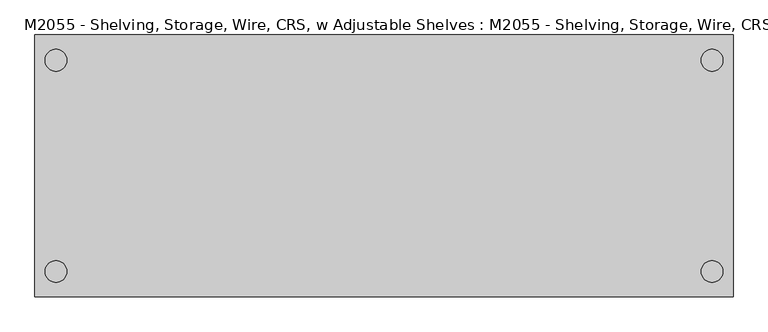
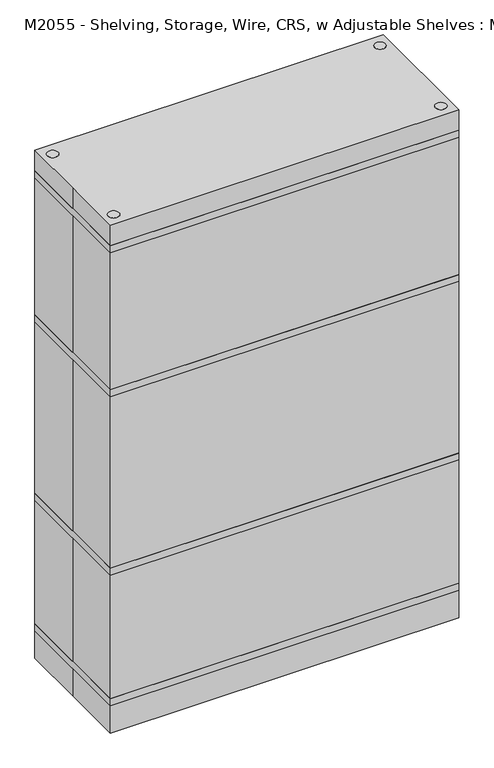
"""IFC4 building model written with IfcOpenShell, lengths in millimetres: proxy geometry, M2055 - Shelving, Storage, Wire, CRS, w Adjustable Shelves : M2055 - Shelving, Storage, Wire, CRS, w Adjustable Shelves."""

import ifcopenshell
import ifcopenshell.guid

model = None  # the IFC model being written
_history = None  # IfcOwnerHistory: only IFC2X3 demands one
_inside = {}  # id of a spatial element -> (the spatial element, [elements in it])
_under = {}  # id of a project, library or spatial element -> (it, [spatial elements below it])
_declared = {}  # id of a project -> (the project, [libraries it declares])
_typed = {}  # id of a type object -> (the type object, [elements of that type])
_made_of = {}  # id of a material, layer set ... -> (it, [elements and type objects made of it])


def new_model(schema):
    """Start an empty IFC model of exactly this schema.

    Asked for "IFC4X3", IfcOpenShell would pick the latest addendum, in which some entities
    have other attributes; the version numbers below select the first issue.
    IFC2X3 requires an IfcOwnerHistory on every rooted entity: one is made here for all.
    """
    global model, _history
    if schema == "IFC4X3":
        model = ifcopenshell.file(schema_version=(4, 3, 0, 0))
    else:
        model = ifcopenshell.file(schema=schema)
    _inside.clear()
    _under.clear()
    _declared.clear()
    _typed.clear()
    _made_of.clear()
    _history = None
    if model.schema == "IFC2X3":
        org = make("IfcOrganization", Name="unknown")
        user = make(
            "IfcPersonAndOrganization",
            ThePerson=make("IfcPerson", FamilyName="unknown"),
            TheOrganization=org,
        )
        app = make(
            "IfcApplication",
            ApplicationDeveloper=org,
            Version="unknown",
            ApplicationFullName="unknown",
            ApplicationIdentifier="unknown",
        )
        _history = make(
            "IfcOwnerHistory",
            OwningUser=user,
            OwningApplication=app,
            ChangeAction="ADDED",
            CreationDate=0,
        )
    return model


def make(cls, **values):
    """One entity of the class cls with the attributes given. An attribute that is None is left unset."""
    return model.create_entity(
        cls, **{name: value for name, value in values.items() if value is not None}
    )


def rooted(cls, **values):
    """An entity with a GlobalId (a new one), such as an element, a storey or a relation."""
    return make(cls, GlobalId=ifcopenshell.guid.new(), OwnerHistory=_history, **values)


def si_unit(unit_type, name, prefix=None):
    """IfcSIUnit, for example si_unit("LENGTHUNIT", "METRE", prefix="MILLI")."""
    return make("IfcSIUnit", UnitType=unit_type, Prefix=prefix, Name=name)


def assignment(units):
    """IfcUnitAssignment: the units of a project."""
    return None if units is None else make("IfcUnitAssignment", Units=units)


def point(xyz):
    """IfcCartesianPoint."""
    return None if xyz is None else make("IfcCartesianPoint", Coordinates=xyz)


def direction(xyz):
    """IfcDirection."""
    return None if xyz is None else make("IfcDirection", DirectionRatios=xyz)


def frame(location, z_axis=None, x_axis=None):
    """IfcAxis2Placement3D, a coordinate frame: its origin and axes. An axis left out is left unset."""
    return make(
        "IfcAxis2Placement3D",
        Location=point(location),
        Axis=direction(z_axis),
        RefDirection=direction(x_axis),
    )


def frame_2d(location, x_axis=None):
    """IfcAxis2Placement2D, a coordinate frame in the plane: its origin and x axis."""
    return make(
        "IfcAxis2Placement2D", Location=point(location), RefDirection=direction(x_axis)
    )


def origin():
    """The frame at (0, 0, 0) with its axes left unset."""
    return frame((0.0, 0.0, 0.0))


def origin_with_axes():
    """The frame at (0, 0, 0) with the z axis (0, 0, 1) and the x axis (1, 0, 0) written out."""
    return frame((0.0, 0.0, 0.0), z_axis=(0.0, 0.0, 1.0), x_axis=(1.0, 0.0, 0.0))


def place(relative_to, where):
    """IfcLocalPlacement: puts the frame where relative to a parent placement (None: the world)."""
    return make(
        "IfcLocalPlacement", PlacementRelTo=relative_to, RelativePlacement=where
    )


def context(
    kind, dimensions, precision=None, world=None, true_north=None, identifier=None
):
    """IfcGeometricRepresentationContext, for example the 3D "Model" context."""
    return make(
        "IfcGeometricRepresentationContext",
        ContextIdentifier=identifier,
        ContextType=kind,
        CoordinateSpaceDimension=dimensions,
        Precision=precision,
        WorldCoordinateSystem=world,
        TrueNorth=true_north,
    )


def project(units=None, contexts=None):
    """IfcProject with its units and contexts."""
    return rooted(
        "IfcProject",
        Name="project",
        RepresentationContexts=contexts,
        UnitsInContext=assignment(units),
    )


def spatial(cls, under=None, at=None, **own):
    """A site, building, storey or space (cls), placed at a placement, below another one or the project."""
    s = rooted(cls, ObjectPlacement=at, **own)
    if under is not None:
        _under.setdefault(under.id(), (under, []))[1].append(s)
    return s


def polyline(points):
    """IfcPolyline through the points."""
    return make("IfcPolyline", Points=[point(p) for p in points])


def circle_curve(where, radius):
    """IfcCircle in the frame where."""
    return make("IfcCircle", Position=where, Radius=radius)


def trimmed(basis, trim1, trim2, sense, master):
    """IfcTrimmedCurve: the piece of a basis curve between two trims."""
    return make(
        "IfcTrimmedCurve",
        BasisCurve=basis,
        Trim1=trim1,
        Trim2=trim2,
        SenseAgreement=sense,
        MasterRepresentation=master,
    )


def segment(curve, same_sense, transition):
    """IfcCompositeCurveSegment."""
    return make(
        "IfcCompositeCurveSegment",
        Transition=transition,
        SameSense=same_sense,
        ParentCurve=curve,
    )


def composite_curve(segments, self_intersect=None):
    """IfcCompositeCurve: segments joined end to end."""
    return make("IfcCompositeCurve", Segments=segments, SelfIntersect=self_intersect)


def outline(outer, holes=None, kind="AREA"):
    """IfcArbitraryClosedProfileDef: a profile drawn as a closed curve; with holes, ...WithVoids."""
    if holes is None:
        return make("IfcArbitraryClosedProfileDef", ProfileType=kind, OuterCurve=outer)
    return make(
        "IfcArbitraryProfileDefWithVoids",
        ProfileType=kind,
        OuterCurve=outer,
        InnerCurves=holes,
    )


def extrude(swept, where, along, depth):
    """IfcExtrudedAreaSolid: the profile swept, set in the frame where, extruded along a direction by depth."""
    return make(
        "IfcExtrudedAreaSolid",
        SweptArea=swept,
        Position=where,
        ExtrudedDirection=direction(along),
        Depth=depth,
    )


def shape(context_of_items, identifier, shape_type, items):
    """IfcShapeRepresentation: the items that make up one representation, for example the "Body"."""
    return make(
        "IfcShapeRepresentation",
        ContextOfItems=context_of_items,
        RepresentationIdentifier=identifier,
        RepresentationType=shape_type,
        Items=items,
    )


def source(mapping_origin, context_of_items, identifier, shape_type, items):
    """IfcRepresentationMap: a shape defined once, which mapped items show again and again."""
    return make(
        "IfcRepresentationMap",
        MappingOrigin=mapping_origin,
        MappedRepresentation=shape(context_of_items, identifier, shape_type, items),
    )


def transform(
    local_origin,
    x_axis=None,
    y_axis=None,
    z_axis=None,
    scale=None,
    scale2=None,
    scale3=None,
    uniform=True,
):
    """IfcCartesianTransformationOperator3D, or its non-uniform kind. x_axis, y_axis, z_axis: its Axis1, 2, 3."""
    if uniform:
        return make(
            "IfcCartesianTransformationOperator3D",
            Axis1=direction(x_axis),
            Axis2=direction(y_axis),
            LocalOrigin=point(local_origin),
            Scale=scale,
            Axis3=direction(z_axis),
        )
    return make(
        "IfcCartesianTransformationOperator3DnonUniform",
        Axis1=direction(x_axis),
        Axis2=direction(y_axis),
        LocalOrigin=point(local_origin),
        Scale=scale,
        Axis3=direction(z_axis),
        Scale2=scale2,
        Scale3=scale3,
    )


def mapped(mapping_source, mapping_target):
    """IfcMappedItem: shows the shape of a source again, moved by a transform."""
    return make(
        "IfcMappedItem", MappingSource=mapping_source, MappingTarget=mapping_target
    )


def made_of(thing, what):
    """Note that an element or type object is made of a material, layer set ...; save() writes the relation."""
    if what is not None:
        _made_of.setdefault(what.id(), (what, []))[1].append(thing)
    return thing


def element(
    cls,
    number,
    at=None,
    inside=None,
    cuts=None,
    type_object=None,
    material=None,
    context=None,
    identifier="Body",
    shape_type=None,
    held_by="IfcProductDefinitionShape",
    body=None,
    shapes=None,
    **own,
):
    """One element of the class cls, such as IfcWall. Its Tag is "e" and its number.

    at: its placement. inside: the storey or other place that contains it. cuts: it is an
    opening in that element (IfcRelVoidsElement). A single representation is given by context,
    identifier, shape_type and body (its items); several are given by shapes. held_by: the class
    of the entity that holds the representations. save() writes the other relations.
    """
    e = rooted(cls, Tag="e%d" % number, ObjectPlacement=at, **own)
    if body is not None:
        shapes = [shape(context, identifier, shape_type, body)]
    if shapes is not None:
        e.Representation = make(held_by, Representations=shapes)
    if inside is not None:
        _inside.setdefault(inside.id(), (inside, []))[1].append(e)
    if cuts is not None:
        rooted(
            "IfcRelVoidsElement", RelatingBuildingElement=cuts, RelatedOpeningElement=e
        )
    if type_object is not None:
        _typed.setdefault(type_object.id(), (type_object, []))[1].append(e)
    return made_of(e, material)


def aggregate(whole, parts):
    """IfcRelAggregates: a whole, such as a stair, and the parts it consists of."""
    return rooted("IfcRelAggregates", RelatingObject=whole, RelatedObjects=parts)


def save(model, path):
    """Write the relations noted so far, then the file.

    IfcRelAggregates (storeys below a building ...), IfcRelContainedInSpatialStructure (elements
    in a storey), IfcRelDefinesByType, IfcRelAssociatesMaterial and IfcRelDeclares: one each for
    every whole, place, type object, material and project.
    """
    for whole, parts in _under.values():
        aggregate(whole, parts)
    for where, things in _inside.values():
        rooted(
            "IfcRelContainedInSpatialStructure",
            RelatedElements=things,
            RelatingStructure=where,
        )
    for kind, things in _typed.values():
        rooted("IfcRelDefinesByType", RelatedObjects=things, RelatingType=kind)
    for what, things in _made_of.values():
        rooted("IfcRelAssociatesMaterial", RelatedObjects=things, RelatingMaterial=what)
    for by, libraries in _declared.values():
        rooted("IfcRelDeclares", RelatingContext=by, RelatedDefinitions=libraries)
    model.write(path)


def m2055_shelving_storage_wire_crs_w_adjustable_shelves_m2055_7b4e6a09(model_context):
    return source(origin(), model_context, "Body", "SweptSolid", [
        extrude(outline(composite_curve([segment(trimmed(circle_curve(frame_2d((572.8672534, -184.4617049)), 19.05), [point((591.9172534, -184.4617049))], [point((553.8172534, -184.4617049))], False, "CARTESIAN"), True, "CONTINUOUS"), segment(trimmed(circle_curve(frame_2d((572.8672534, -184.4617049)), 19.05), [point((553.8172534, -184.4617049))], [point((591.9172534, -184.4617049))], False, "CARTESIAN"), True, "CONTINUOUS")], self_intersect=False)), origin_with_axes(), (0.0, 0.0, 1.0), 1879.6),
        extrude(outline(composite_curve([segment(trimmed(circle_curve(frame_2d((-572.8672534, -184.4617049)), 19.05), [point((-591.9172534, -184.4617049))], [point((-553.8172534, -184.4617049))], False, "CARTESIAN"), True, "CONTINUOUS"), segment(trimmed(circle_curve(frame_2d((-572.8672534, -184.4617049)), 19.05), [point((-553.8172534, -184.4617049))], [point((-591.9172534, -184.4617049))], False, "CARTESIAN"), True, "CONTINUOUS")], self_intersect=False)), origin_with_axes(), (0.0, 0.0, 1.0), 1879.6),
        extrude(outline(composite_curve([segment(trimmed(circle_curve(frame_2d((572.8672534, 184.4617049)), 19.05), [point((591.9172534, 184.4617049))], [point((553.8172534, 184.4617049))], False, "CARTESIAN"), True, "CONTINUOUS"), segment(trimmed(circle_curve(frame_2d((572.8672534, 184.4617049)), 19.05), [point((553.8172534, 184.4617049))], [point((591.9172534, 184.4617049))], False, "CARTESIAN"), True, "CONTINUOUS")], self_intersect=False)), origin_with_axes(), (0.0, 0.0, 1.0), 1879.6),
        extrude(outline(composite_curve([segment(trimmed(circle_curve(frame_2d((-572.8672534, 184.4617049)), 19.05), [point((-591.9172534, 184.4617049))], [point((-553.8172534, 184.4617049))], False, "CARTESIAN"), True, "CONTINUOUS"), segment(trimmed(circle_curve(frame_2d((-572.8672534, 184.4617049)), 19.05), [point((-553.8172534, 184.4617049))], [point((-591.9172534, 184.4617049))], False, "CARTESIAN"), True, "CONTINUOUS")], self_intersect=False)), origin_with_axes(), (0.0, 0.0, 1.0), 1879.6),
        extrude(outline(polyline([(609.6, 228.6), (609.6, -228.6), (-609.6, -228.6), (-609.6, 228.6), (609.6, 228.6)])), frame((0.0, 0.0, 1778.0), z_axis=(0.0, 0.0, 1.0), x_axis=(1.0, 0.0, 0.0)), (0.0, 0.0, 1.0), 25.4),
        extrude(outline(polyline([(609.6, 228.6), (609.6, -228.6), (-609.6, -228.6), (-609.6, 228.6), (609.6, 228.6)])), frame((0.0, 0.0, 1244.6), z_axis=(0.0, 0.0, 1.0), x_axis=(1.0, 0.0, 0.0)), (0.0, 0.0, 1.0), 25.4),
        extrude(outline(polyline([(609.6, 228.6), (609.6, -228.6), (-609.6, -228.6), (-609.6, 228.6), (609.6, 228.6)])), frame((0.0, 0.0, 584.2), z_axis=(0.0, 0.0, 1.0), x_axis=(1.0, 0.0, 0.0)), (0.0, 0.0, 1.0), 25.4),
        extrude(outline(polyline([(609.6, 228.6), (609.6, -228.6), (-609.6, -228.6), (-609.6, 228.6), (609.6, 228.6)])), frame((0.0, 0.0, 101.6), z_axis=(0.0, 0.0, 1.0), x_axis=(1.0, 0.0, 0.0)), (0.0, 0.0, 1.0), 25.4),
        extrude(outline(polyline([(-609.6, 228.6), (609.6, 228.6), (609.6, -228.6), (-609.6, -228.6), (-609.6, 0.0), (-609.6, 228.6)])), origin_with_axes(), (0.0, 0.0, 1.0), 1879.6),
    ])


if __name__ == "__main__":
    model = new_model("IFC4")
    model_context = context("Model", 3, world=origin())
    ifc_project = project(units=[si_unit("LENGTHUNIT", "METRE", prefix="MILLI")], contexts=[model_context])
    site = spatial("IfcSite", under=ifc_project)
    building = spatial("IfcBuilding", under=site)
    placement = place(None, origin())
    m2055_shelving_storage_wire_crs_w_adjustable_shelves_m2055_shape = m2055_shelving_storage_wire_crs_w_adjustable_shelves_m2055_7b4e6a09(model_context)
    element("IfcBuildingElementProxy", 1, Name="M2055 - Shelving, Storage, Wire, CRS, w Adjustable Shelves : M2055 - Shelving, Storage, Wire, CRS, w Adjustable Shelves", ObjectType="M2055 - Shelving, Storage, Wire, CRS, w Adjustable Shelves : M2055 - Shelving, Storage, Wire, CRS, w Adjustable Shelves", at=placement, inside=building, context=model_context, shape_type="MappedRepresentation", body=[
        mapped(m2055_shelving_storage_wire_crs_w_adjustable_shelves_m2055_shape, transform((0.0, 0.0, 0.0), x_axis=(1.0, 0.0, 0.0), y_axis=(0.0, 1.0, 0.0), z_axis=(0.0, 0.0, 1.0))),
    ])
    save(model, "model.ifc")

# Revit data of these elements
# Type "M2055 - Shelving, Storage, Wire, CRS, w Adjustable Shelves : M2055 - Shelving, Storage, Wire, CRS, w Adjustable Shelves"
#   Watts2 = "0"
#   Watts1 = "0"
#   Unit_Issue = "EA"
#   UTIL_6_Misc = "-"
#   UTIL_5_NonMedGas = "-"
#   UTIL_4_MiscGas = "-"
#   UTIL_3_MedGas = "-"
#   UTIL_2_Elec = "-"
#   UTIL_1_WaterDrain = "-"
#   Nomenclature = "Shelving, Storage, Wire, CRS, w/Adjustable Shelves"
#   NSN = "7100"
#   Location [instance default] = ""
#   JSN = "M2055"
#   Fund_Source_VA = "-"
#   Fund_Source_Navy = "-"
#   Fund_Source_Army = "-"
#   Fund_Source_AF = "-"
#   ELEC_Volts2 = "0"
#   ELEC_Volts1 = "0"
#   ELEC_Phase2 = "0"
#   ELEC_Phase1 = "0"
#   ELEC_HertzSwitch = "0"
#   ELEC_HertzDependent = "0"
#   ELEC_Hertz = "0"
#   ELEC_Amps2 = "0"
#   ELEC_Amps1 = "0"
#   DetailDescription = "Stationary, wire, shelving unit. Unit has fully adjustable shelves constructed of stainless steel. For use in general purpose storage areas. Shelving is provided in various sizes and configurations. Price provided is for a unit approximately 74\"H x 18\"D x 48\"W with four shelves."
#   CAT_VA = "C"
#   CAT_Navy = "C"
#   CAT_IHS = "-"
#   CAT_Army = "C"
#   CAT_AF = "C"
#   BTUperhour = "0"
#   Weight_IP = 80
#   DIM_Width_IP = 4' - 0"
#   DIM_Height_IP = 6' - 2"
#   DIM_Depth_IP = 1' - 6"
# Element 1 (IfcBuildingElementProxy, "M2055 - Shelving, Storage, Wire, CRS, w Adjustable Shelves : M2055 - Shelving, Storage, Wire, CRS, w Adjustable Shelves")
#   Materials on its faces: "EquipSpace"
# Materials
#   "EquipSpace": class "Unassigned", colour RGB 221 217 195, transparency 0.5
